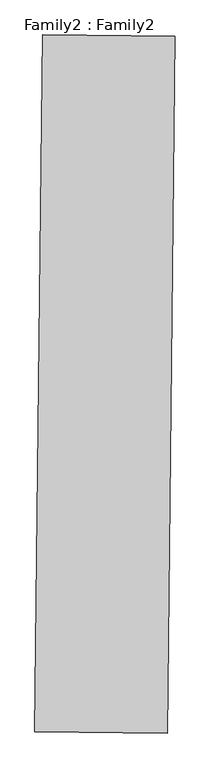
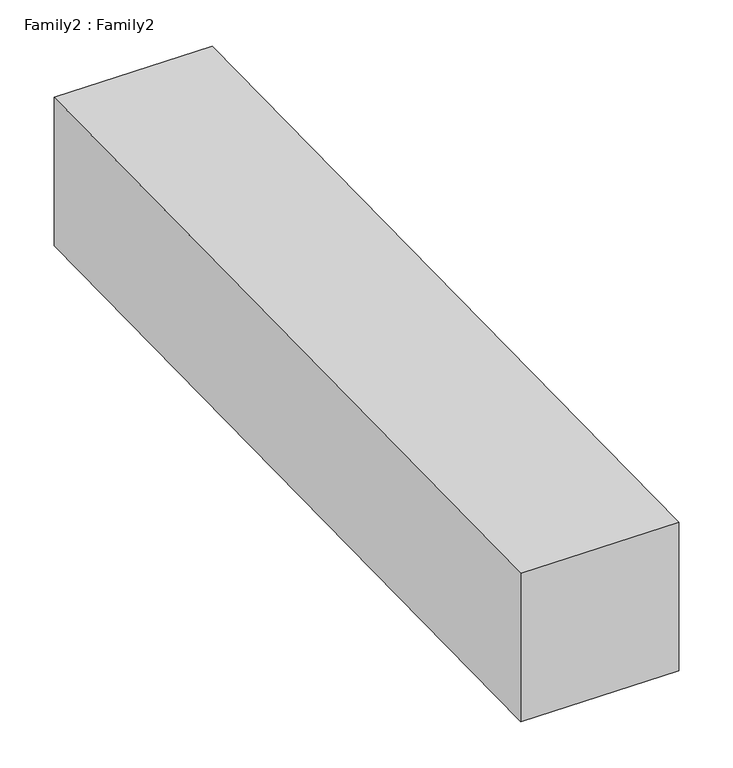
"""IFC4 building model written with IfcOpenShell, lengths in millimetres: proxy geometry, Family2 : Family2."""

from ifc_helpers import new_model, si_unit, origin, place, context, project, spatial, faceted_brep, source, transform, mapped, element, save


def family2_family2_d1389313(model_context):
    return source(origin(), model_context, "Body", "Brep", [
        faceted_brep([(-3949.1556602, -6597.9254493, 1.0945136), (-3949.1556602, -6597.9254493, 201.0945136), (-3937.6871343, -5549.6746733, 202.060409), (-3937.6871343, -5549.6746733, 2.060409), (-3749.1644702, -6599.8026619, 201.0945136), (-3737.6959444, -5551.551886, 202.060409), (-3749.1644702, -6599.8026619, 1.0945136), (-3737.6959444, -5551.551886, 2.060409)], [[[0, 1, 2, 3]], [[1, 4, 5, 2]], [[4, 6, 7, 5]], [[6, 0, 3, 7]], [[3, 2, 5, 7]], [[0, 6, 4, 1]]]),
    ])


if __name__ == "__main__":
    model = new_model("IFC4")
    model_context = context("Model", 3, world=origin())
    ifc_project = project(units=[si_unit("LENGTHUNIT", "METRE", prefix="MILLI")], contexts=[model_context])
    site = spatial("IfcSite", under=ifc_project)
    building = spatial("IfcBuilding", under=site)
    placement = place(None, origin())
    family2_family2_shape = family2_family2_d1389313(model_context)
    element("IfcBuildingElementProxy", 1, Name="Family2 : Family2", ObjectType="Family2 : Family2", at=placement, inside=building, context=model_context, shape_type="MappedRepresentation", body=[
        mapped(family2_family2_shape, transform((0.0, 0.0, 0.0), x_axis=(1.0, 0.0, 0.0), y_axis=(0.0, 1.0, 0.0), z_axis=(0.0, 0.0, 1.0))),
    ])
    save(model, "model.ifc")

# Revit data of these elements
# Type "Family2 : Family2"
#   Default Elevation = 0
